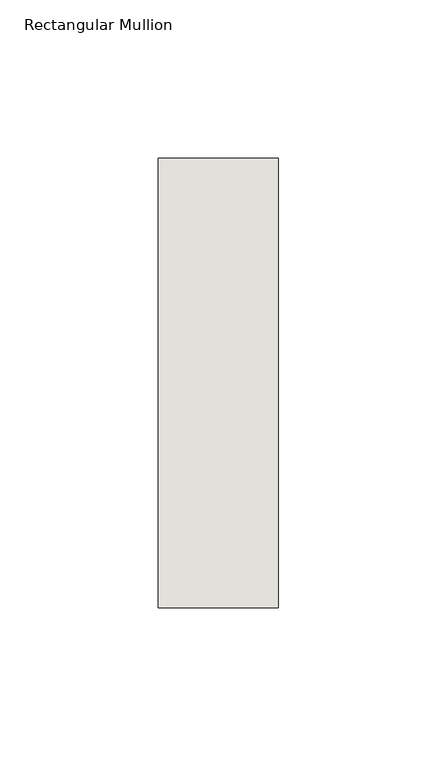
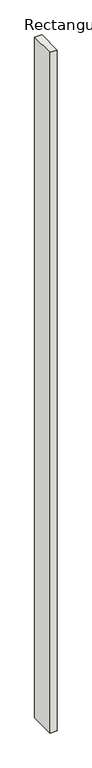
"""IFC4 building model written with IfcOpenShell, lengths in millimetres: wall geometry, Rectangular Mullion : NLRS_21_CWM_hsb-regel 38x142_gen_rsf."""

from ifc_helpers import new_model, si_unit, frame, origin, place, context, project, spatial, polyline, outline, extrude, source, transform, mapped, element, save


def rectangular_mullion_d78042b4(model_context):
    return source(origin(), model_context, "Body", "SweptSolid", [
        extrude(outline(polyline([(-38.0, -71.0), (-38.0, 71.0), (0.0, 71.0), (0.0, -71.0), (-38.0, -71.0)])), frame((0.0, 0.0, -3849.0), z_axis=(0.0, 0.0, 1.0), x_axis=(1.0, 0.0, 0.0)), (0.0, 0.0, 1.0), 3849.0),
    ])


if __name__ == "__main__":
    model = new_model("IFC4")
    model_context = context("Model", 3, world=origin())
    ifc_project = project(units=[si_unit("LENGTHUNIT", "METRE", prefix="MILLI")], contexts=[model_context])
    site = spatial("IfcSite", under=ifc_project)
    building = spatial("IfcBuilding", under=site)
    placement = place(None, origin())
    rectangular_mullion_shape = rectangular_mullion_d78042b4(model_context)
    element("IfcWall", 1, ObjectType="Rectangular Mullion : NLRS_21_CWM_hsb-regel 38x142_gen_rsf", at=placement, inside=building, context=model_context, shape_type="MappedRepresentation", body=[
        mapped(rectangular_mullion_shape, transform((0.0, 0.0, 0.0), x_axis=(1.0, 0.0, 0.0), y_axis=(0.0, 1.0, 0.0), z_axis=(0.0, 0.0, 1.0))),
    ])
    save(model, "model.ifc")

# Revit data of these elements
# Type "Rectangular Mullion : NLRS_21_CWM_hsb-regel 38x142_gen_rsf"
#   Type IfcGUID = "07M7mRoiH1CR8m_RSKIwpF"
#   Assembly Code = "21.10"
#   IfcExportAs = "IfcWall"
#   built-in parameter 1007322 = 0.465879 (stored number, unit not read)
#   built-in parameter 1007321 = 0.062336 (stored number, unit not read)
#   built-in parameter 1007320 = 0.062336 (stored number, unit not read)
# Element 1 (IfcWall, "Rectangular Mullion : NLRS_21_CWM_hsb-regel 38x142_gen_rsf")
#   Materials on its faces: "NLRS_i2_hout naaldhout vuren_gen_rsf"
# Materials
#   "NLRS_i2_hout naaldhout vuren_gen_rsf": class "I - Hout", colour RGB 234 199 147, transparency 0, Keynote = "i2", Manufacturer = "Revit Standards Foundation", URL = "www.revitstandards.org", Description = "hout vuren", Cost = 0
